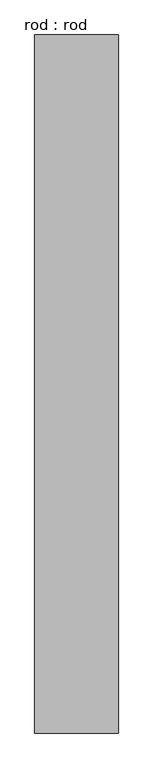
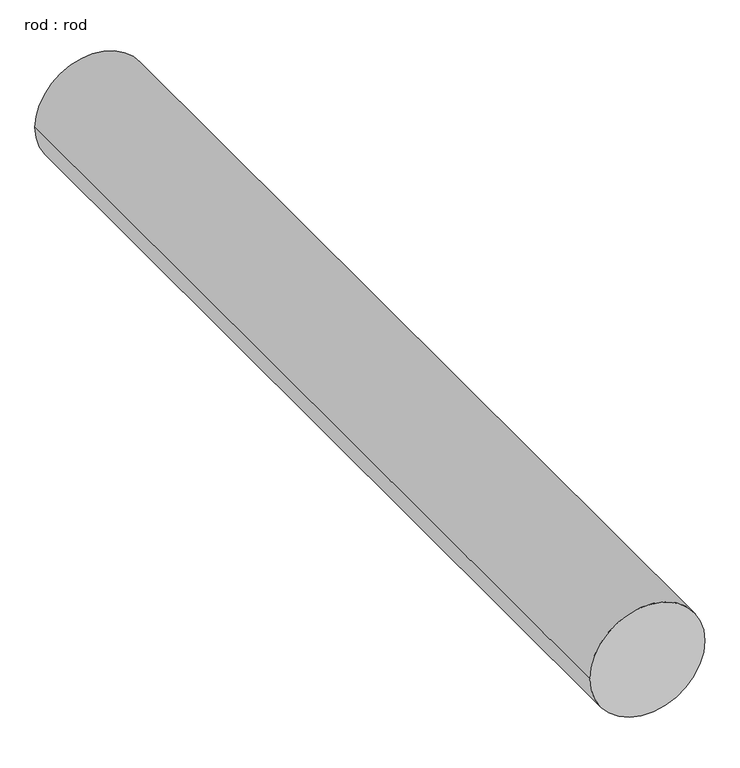
"""IFC4 building model written with IfcOpenShell, lengths in millimetres: proxy geometry, rod : rod."""

from ifc_helpers import new_model, si_unit, point, frame, frame_2d, origin, place, context, project, spatial, circle_curve, trimmed, segment, composite_curve, outline, extrude, source, transform, mapped, element, save


def rod_rod_572fcbe8(model_context):
    return source(origin(), model_context, "Body", "SweptSolid", [
        extrude(outline(composite_curve([segment(trimmed(circle_curve(frame_2d((0.0108462, 0.0)), 200.0), [point((0.0108462, 200.0))], [point((0.0108462, -200.0))], False, "CARTESIAN"), True, "CONTINUOUS"), segment(trimmed(circle_curve(frame_2d((0.0108462, 0.0)), 200.0), [point((0.0108462, -200.0))], [point((0.0108462, 200.0))], False, "CARTESIAN"), True, "CONTINUOUS")], self_intersect=False)), frame((0.0, 2422.7286153, 0.0), z_axis=(0.0, 1.0, 0.0), x_axis=(0.0, 0.0, 1.0)), (0.0, 0.0, 1.0), 3340.0),
    ])


if __name__ == "__main__":
    model = new_model("IFC4")
    model_context = context("Model", 3, world=origin())
    ifc_project = project(units=[si_unit("LENGTHUNIT", "METRE", prefix="MILLI")], contexts=[model_context])
    site = spatial("IfcSite", under=ifc_project)
    building = spatial("IfcBuilding", under=site)
    placement = place(None, origin())
    rod_rod_shape = rod_rod_572fcbe8(model_context)
    element("IfcBuildingElementProxy", 1, Name="rod : rod", ObjectType="rod : rod", at=placement, inside=building, context=model_context, shape_type="MappedRepresentation", body=[
        mapped(rod_rod_shape, transform((0.0, 0.0, 0.0), x_axis=(1.0, 0.0, 0.0), y_axis=(0.0, 1.0, 0.0), z_axis=(0.0, 0.0, 1.0))),
    ])
    save(model, "model.ifc")

# Revit data of these elements
# Type "rod : rod"
#   Default Elevation = 0
